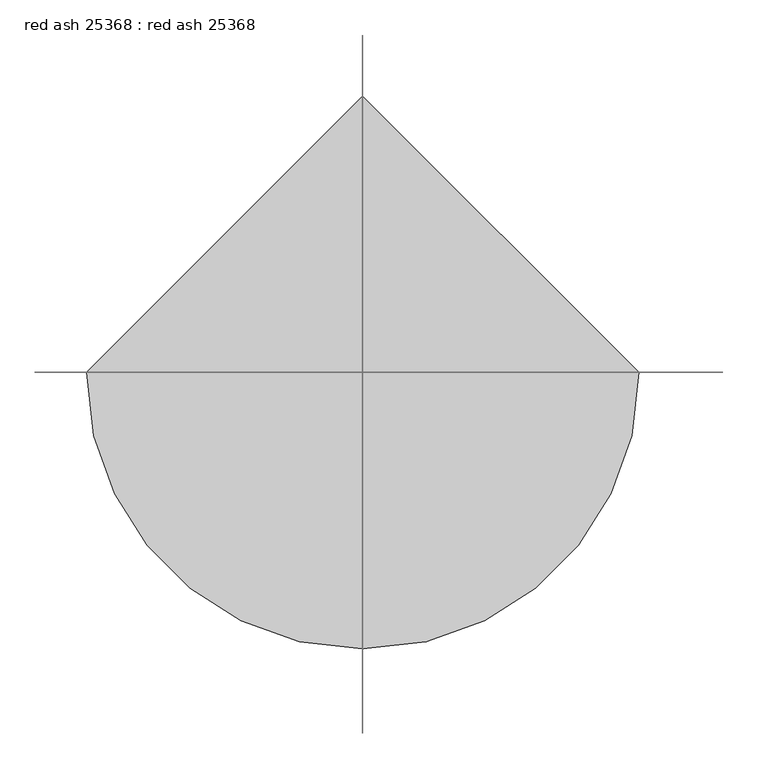
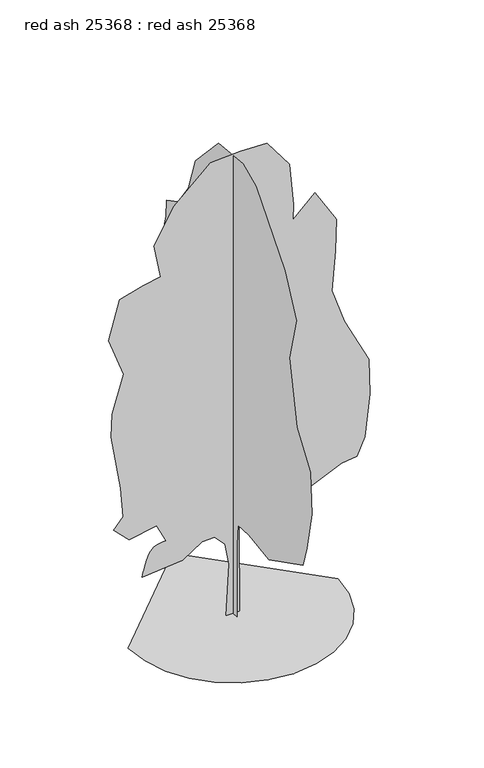
"""IFC4 building model written with IfcOpenShell, lengths in millimetres: proxy geometry, red ash 25368 : red ash 25368."""

import ifcopenshell
import ifcopenshell.guid

model = None  # the IFC model being written
_history = None  # IfcOwnerHistory: only IFC2X3 demands one
_inside = {}  # id of a spatial element -> (the spatial element, [elements in it])
_under = {}  # id of a project, library or spatial element -> (it, [spatial elements below it])
_declared = {}  # id of a project -> (the project, [libraries it declares])
_typed = {}  # id of a type object -> (the type object, [elements of that type])
_made_of = {}  # id of a material, layer set ... -> (it, [elements and type objects made of it])


def new_model(schema):
    """Start an empty IFC model of exactly this schema.

    Asked for "IFC4X3", IfcOpenShell would pick the latest addendum, in which some entities
    have other attributes; the version numbers below select the first issue.
    IFC2X3 requires an IfcOwnerHistory on every rooted entity: one is made here for all.
    """
    global model, _history
    if schema == "IFC4X3":
        model = ifcopenshell.file(schema_version=(4, 3, 0, 0))
    else:
        model = ifcopenshell.file(schema=schema)
    _inside.clear()
    _under.clear()
    _declared.clear()
    _typed.clear()
    _made_of.clear()
    _history = None
    if model.schema == "IFC2X3":
        org = make("IfcOrganization", Name="unknown")
        user = make(
            "IfcPersonAndOrganization",
            ThePerson=make("IfcPerson", FamilyName="unknown"),
            TheOrganization=org,
        )
        app = make(
            "IfcApplication",
            ApplicationDeveloper=org,
            Version="unknown",
            ApplicationFullName="unknown",
            ApplicationIdentifier="unknown",
        )
        _history = make(
            "IfcOwnerHistory",
            OwningUser=user,
            OwningApplication=app,
            ChangeAction="ADDED",
            CreationDate=0,
        )
    return model


def make(cls, **values):
    """One entity of the class cls with the attributes given. An attribute that is None is left unset."""
    return model.create_entity(
        cls, **{name: value for name, value in values.items() if value is not None}
    )


def rooted(cls, **values):
    """An entity with a GlobalId (a new one), such as an element, a storey or a relation."""
    return make(cls, GlobalId=ifcopenshell.guid.new(), OwnerHistory=_history, **values)


def si_unit(unit_type, name, prefix=None):
    """IfcSIUnit, for example si_unit("LENGTHUNIT", "METRE", prefix="MILLI")."""
    return make("IfcSIUnit", UnitType=unit_type, Prefix=prefix, Name=name)


def assignment(units):
    """IfcUnitAssignment: the units of a project."""
    return None if units is None else make("IfcUnitAssignment", Units=units)


def point(xyz):
    """IfcCartesianPoint."""
    return None if xyz is None else make("IfcCartesianPoint", Coordinates=xyz)


def direction(xyz):
    """IfcDirection."""
    return None if xyz is None else make("IfcDirection", DirectionRatios=xyz)


def frame(location, z_axis=None, x_axis=None):
    """IfcAxis2Placement3D, a coordinate frame: its origin and axes. An axis left out is left unset."""
    return make(
        "IfcAxis2Placement3D",
        Location=point(location),
        Axis=direction(z_axis),
        RefDirection=direction(x_axis),
    )


def origin():
    """The frame at (0, 0, 0) with its axes left unset."""
    return frame((0.0, 0.0, 0.0))


def place(relative_to, where):
    """IfcLocalPlacement: puts the frame where relative to a parent placement (None: the world)."""
    return make(
        "IfcLocalPlacement", PlacementRelTo=relative_to, RelativePlacement=where
    )


def context(
    kind, dimensions, precision=None, world=None, true_north=None, identifier=None
):
    """IfcGeometricRepresentationContext, for example the 3D "Model" context."""
    return make(
        "IfcGeometricRepresentationContext",
        ContextIdentifier=identifier,
        ContextType=kind,
        CoordinateSpaceDimension=dimensions,
        Precision=precision,
        WorldCoordinateSystem=world,
        TrueNorth=true_north,
    )


def project(units=None, contexts=None):
    """IfcProject with its units and contexts."""
    return rooted(
        "IfcProject",
        Name="project",
        RepresentationContexts=contexts,
        UnitsInContext=assignment(units),
    )


def spatial(cls, under=None, at=None, **own):
    """A site, building, storey or space (cls), placed at a placement, below another one or the project."""
    s = rooted(cls, ObjectPlacement=at, **own)
    if under is not None:
        _under.setdefault(under.id(), (under, []))[1].append(s)
    return s


def point_list(points):
    """IfcCartesianPointList2D or 3D."""
    cls = (
        "IfcCartesianPointList2D" if len(points[0]) == 2 else "IfcCartesianPointList3D"
    )
    return make(cls, CoordList=points)


def triangles(points, corners, closed=None, point_numbers=None):
    """IfcTriangulatedFaceSet: each triangle names its three corners, points numbered from 1."""
    return make(
        "IfcTriangulatedFaceSet",
        Coordinates=point_list(points),
        Closed=closed,
        CoordIndex=corners,
        PnIndex=point_numbers,
    )


def shape(context_of_items, identifier, shape_type, items):
    """IfcShapeRepresentation: the items that make up one representation, for example the "Body"."""
    return make(
        "IfcShapeRepresentation",
        ContextOfItems=context_of_items,
        RepresentationIdentifier=identifier,
        RepresentationType=shape_type,
        Items=items,
    )


def source(mapping_origin, context_of_items, identifier, shape_type, items):
    """IfcRepresentationMap: a shape defined once, which mapped items show again and again."""
    return make(
        "IfcRepresentationMap",
        MappingOrigin=mapping_origin,
        MappedRepresentation=shape(context_of_items, identifier, shape_type, items),
    )


def transform(
    local_origin,
    x_axis=None,
    y_axis=None,
    z_axis=None,
    scale=None,
    scale2=None,
    scale3=None,
    uniform=True,
):
    """IfcCartesianTransformationOperator3D, or its non-uniform kind. x_axis, y_axis, z_axis: its Axis1, 2, 3."""
    if uniform:
        return make(
            "IfcCartesianTransformationOperator3D",
            Axis1=direction(x_axis),
            Axis2=direction(y_axis),
            LocalOrigin=point(local_origin),
            Scale=scale,
            Axis3=direction(z_axis),
        )
    return make(
        "IfcCartesianTransformationOperator3DnonUniform",
        Axis1=direction(x_axis),
        Axis2=direction(y_axis),
        LocalOrigin=point(local_origin),
        Scale=scale,
        Axis3=direction(z_axis),
        Scale2=scale2,
        Scale3=scale3,
    )


def mapped(mapping_source, mapping_target):
    """IfcMappedItem: shows the shape of a source again, moved by a transform."""
    return make(
        "IfcMappedItem", MappingSource=mapping_source, MappingTarget=mapping_target
    )


def made_of(thing, what):
    """Note that an element or type object is made of a material, layer set ...; save() writes the relation."""
    if what is not None:
        _made_of.setdefault(what.id(), (what, []))[1].append(thing)
    return thing


def element(
    cls,
    number,
    at=None,
    inside=None,
    cuts=None,
    type_object=None,
    material=None,
    context=None,
    identifier="Body",
    shape_type=None,
    held_by="IfcProductDefinitionShape",
    body=None,
    shapes=None,
    **own,
):
    """One element of the class cls, such as IfcWall. Its Tag is "e" and its number.

    at: its placement. inside: the storey or other place that contains it. cuts: it is an
    opening in that element (IfcRelVoidsElement). A single representation is given by context,
    identifier, shape_type and body (its items); several are given by shapes. held_by: the class
    of the entity that holds the representations. save() writes the other relations.
    """
    e = rooted(cls, Tag="e%d" % number, ObjectPlacement=at, **own)
    if body is not None:
        shapes = [shape(context, identifier, shape_type, body)]
    if shapes is not None:
        e.Representation = make(held_by, Representations=shapes)
    if inside is not None:
        _inside.setdefault(inside.id(), (inside, []))[1].append(e)
    if cuts is not None:
        rooted(
            "IfcRelVoidsElement", RelatingBuildingElement=cuts, RelatedOpeningElement=e
        )
    if type_object is not None:
        _typed.setdefault(type_object.id(), (type_object, []))[1].append(e)
    return made_of(e, material)


def aggregate(whole, parts):
    """IfcRelAggregates: a whole, such as a stair, and the parts it consists of."""
    return rooted("IfcRelAggregates", RelatingObject=whole, RelatedObjects=parts)


def save(model, path):
    """Write the relations noted so far, then the file.

    IfcRelAggregates (storeys below a building ...), IfcRelContainedInSpatialStructure (elements
    in a storey), IfcRelDefinesByType, IfcRelAssociatesMaterial and IfcRelDeclares: one each for
    every whole, place, type object, material and project.
    """
    for whole, parts in _under.values():
        aggregate(whole, parts)
    for where, things in _inside.values():
        rooted(
            "IfcRelContainedInSpatialStructure",
            RelatedElements=things,
            RelatingStructure=where,
        )
    for kind, things in _typed.values():
        rooted("IfcRelDefinesByType", RelatedObjects=things, RelatingType=kind)
    for what, things in _made_of.values():
        rooted("IfcRelAssociatesMaterial", RelatedObjects=things, RelatingMaterial=what)
    for by, libraries in _declared.values():
        rooted("IfcRelDeclares", RelatingContext=by, RelatedDefinitions=libraries)
    model.write(path)


def red_ash_25368_red_ash_25368_14781bec(model_context):
    return source(origin(), model_context, "Body", "Tessellation", [
        triangles([(-1644.9525009, 0.0, 6.19e-05), (-1601.4651844, -376.9143482, 6.19e-05), (-1477.6144592, -723.0498339, 6.19e-05), (-1283.3164352, -1028.4894024, 6.19e-05), (-1028.4894751, -1283.3165806, 6.19e-05), (-723.0496885, -1477.6140232, 6.19e-05), (-376.9141665, -1601.4651844, 6.19e-05), (7.19e-05, -1644.9525009, 6.19e-05), (376.9143846, -1601.4651844, 6.19e-05), (723.0499065, -1477.6143139, 6.19e-05), (1028.4894751, -1283.3164352, 6.19e-05), (1283.3168713, -1028.4894751, 6.19e-05), (1477.6141685, -723.0496159, 6.19e-05), (1601.4651844, -376.9140939, 6.19e-05), (1644.9525009, 0.0001438, 6.19e-05), (-0.0002157, 1644.9525009, 6.19e-05), (-1.07e-05, -102.8462569, 0.0), (2.5e-05, -101.2467179, 1194.554048), (3.23e-05, -129.8819613, 1537.8029366), (7e-07, -438.8253948, 1558.1655018), (-5.78e-05, -976.3912743, 1478.3068588), (-0.0001405, -1903.692667, 1948.6771305), (-0.0001413, -2011.2060173, 2298.095192), (-0.0001361, -2145.5975235, 2943.1744217), (-0.0001119, -2105.2803623, 3615.1319527), (-5.81e-05, -1740.3819958, 4141.0172951), (-5.5e-06, -1527.3986298, 5160.6350006), (-3.5e-06, -1715.5451397, 5886.3488434), (4.79e-05, -1406.4449661, 6531.4286545), (0.0001569, -626.9743755, 7458.7301926), (0.0001985, -273.2007115, 7618.1942963), (0.0002662, 394.4016166, 7552.8046829), (0.0003121, 1026.0418774, 6880.8468613), (0.0003149, 1214.190204, 6316.4022446), (0.0003323, 1496.411277, 5913.2274353), (0.0003598, 1805.5131947, 5751.9582092), (0.0003531, 1818.9521999, 5483.1746155), (0.0003523, 1899.587249, 5174.0742966), (0.0003275, 1765.1957428, 4811.2170845), (0.0003297, 1886.1480984, 4461.7991684), (0.0003279, 2007.1004539, 3977.9897461), (0.0003211, 1980.222298, 3843.5979492), (0.0002877, 1751.7567375, 3521.0580437), (0.0002729, 1737.3115437, 3077.5662186), (0.0002632, 1724.8782909, 2795.3439102), (0.0002542, 1738.3174416, 2445.9262848), (0.0002412, 1751.7568829, 1962.1167171), (0.0002172, 1563.6084835, 1814.2857697), (0.0001807, 1214.1907127, 1814.2857697), (0.0001827, 1375.4605202, 1317.0371967), (0.0001715, 1348.4951603, 1034.8845062), (0.0001516, 1103.0310734, 1227.8363914), (9.86e-05, 629.4626684, 1106.7075932), (9.8e-05, 551.7118183, 1357.0609165), (6.29e-05, 215.9127657, 1354.0025276), (5.03e-05, 130.8012366, 1228.3346169), (3.27e-05, 79.5493323, 818.2831198), (1.17e-05, 112.1660096, 1.28e-05), (-110.870867, 4.8e-06, 4.46e-05), (-66.7114758, -9.64e-05, 833.5016676), (-129.3072962, -0.000136, 1187.9435503), (-290.7878647, -0.00015, 1365.31768), (-483.6364677, -0.0001408, 1358.6964272), (-796.2678211, -0.000103, 1155.7673166), (-1427.9080456, -6.9e-05, 1102.0108595), (-1419.1706429, -7.35e-05, 1136.7646975), (-1409.8454853, -7.82e-05, 1172.6938271), (-1399.3449635, -8.32e-05, 1210.9736853), (-1387.0813225, -8.87e-05, 1252.7803631), (-1372.4668076, -9.49e-05, 1299.2876987), (-1354.9136639, -0.0001019, 1351.6733093), (-1333.8341366, -0.0001099, 1411.1111057), (-1307.2693336, -0.0001176, 1466.2392815), (-1274.3570984, -0.0001239, 1506.556588), (-1236.1555058, -0.0001289, 1534.5316246), (-1193.7220493, -0.0001329, 1552.6338627), (-1148.1152401, -0.0001362, 1563.3300121), (-1100.3923536, -0.000139, 1569.0895443), (-1051.6116829, -0.0001415, 1572.3809132), (-1199.4421944, -0.0001703, 1868.0423721), (-1629.4953049, -0.0001418, 1787.4073231), (-1871.3997253, -0.0001601, 2029.3124702), (-1723.5690685, -0.0001874, 2204.0214283), (-1763.886375, -0.0002433, 2687.8309959), (-1911.7170319, -0.0003442, 3588.2539421), (-1898.4807758, -0.0003892, 3961.1654823), (-1719.9175472, -0.0004688, 4563.3255295), (-1952.0346291, -0.0005347, 5200.9523071), (-1777.3253803, -0.000616, 5819.1535263), (-1414.4687496, -0.0006447, 5926.6667313), (-1138.413216, -0.0006626, 5975.3625961), (-1239.7599369, -0.0007228, 6517.9893585), (-930.6591093, -0.000802, 7068.9952606), (-352.7753057, -0.0008898, 7593.1219894), (117.5946844, -0.0009135, 7620.0), (534.2087442, -0.0009301, 7606.5601227), (883.626733, -0.0008893, 7136.1905777), (947.8720848, -0.00081, 6447.5180786), (938.6469212, -0.0007795, 6194.9695404), (1286.8011063, -0.0008333, 6517.9893585), (1622.7800171, -0.0007823, 5966.9840378), (1609.3410118, -0.0007196, 5446.5094116), (1549.4574577, -0.00064, 4800.6520317), (1743.7323727, -0.0005809, 4233.3331718), (2131.7640656, -0.0005067, 3469.1978371), (2144.1354034, -0.0004386, 2892.8094727), (2066.2719875, -0.0003531, 2204.021283), (1945.319632, -0.0003141, 1921.7989746), (1703.4147755, -0.0003004, 1894.9206734), (1233.0446491, -0.0002542, 1679.8941181), (816.4305439, -0.0002007, 1384.2328045), (257.4765441, -0.0002049, 1624.5688614), (93.0508701, -0.0001766, 1447.6347485), (104.1552431, -4.6e-06, 3.52e-05)], [[15, 16, 1], [14, 15, 1], [14, 1, 2], [13, 14, 2], [13, 2, 3], [13, 3, 4], [12, 13, 4], [11, 12, 4], [11, 4, 5], [11, 5, 6], [11, 6, 7], [11, 7, 8], [11, 8, 9], [11, 9, 10], [50, 51, 52], [57, 58, 17], [57, 17, 18], [56, 57, 18], [56, 18, 19], [55, 56, 19], [49, 50, 52], [52, 53, 54], [49, 52, 54], [35, 36, 37], [46, 47, 48], [46, 48, 49], [21, 22, 23], [20, 21, 23], [20, 23, 24], [20, 24, 25], [20, 25, 26], [19, 20, 26], [19, 26, 27], [45, 46, 49], [31, 32, 33], [30, 31, 33], [29, 30, 33], [29, 33, 34], [28, 29, 34], [27, 28, 34], [19, 27, 34], [19, 34, 35], [19, 35, 37], [19, 37, 38], [19, 38, 39], [19, 39, 40], [19, 40, 41], [19, 41, 42], [19, 42, 43], [19, 43, 44], [19, 44, 45], [19, 45, 49], [19, 49, 54], [55, 19, 54], [64, 65, 66], [64, 66, 67], [64, 67, 68], [99, 100, 101], [64, 68, 69], [64, 69, 70], [64, 70, 71], [114, 59, 60], [113, 114, 60], [113, 60, 61], [113, 61, 62], [64, 71, 72], [64, 72, 73], [64, 73, 74], [64, 74, 75], [64, 75, 76], [64, 76, 77], [64, 77, 78], [64, 78, 79], [63, 64, 79], [81, 82, 83], [80, 81, 83], [99, 101, 102], [107, 108, 109], [110, 111, 112], [88, 89, 90], [87, 88, 90], [87, 90, 91], [80, 83, 84], [95, 96, 97], [95, 97, 98], [94, 95, 98], [93, 94, 98], [92, 93, 98], [91, 92, 98], [91, 98, 99], [87, 91, 99], [87, 99, 102], [87, 102, 103], [87, 103, 104], [86, 87, 104], [85, 86, 104], [84, 85, 104], [80, 84, 104], [80, 104, 105], [80, 105, 106], [80, 106, 107], [80, 107, 109], [80, 109, 110], [80, 110, 112], [79, 80, 112], [63, 79, 112], [62, 63, 112], [113, 62, 112]], closed=False),
    ])


if __name__ == "__main__":
    model = new_model("IFC4")
    model_context = context("Model", 3, world=origin())
    ifc_project = project(units=[si_unit("LENGTHUNIT", "METRE", prefix="MILLI")], contexts=[model_context])
    site = spatial("IfcSite", under=ifc_project)
    building = spatial("IfcBuilding", under=site)
    placement = place(None, origin())
    red_ash_25368_red_ash_25368_shape = red_ash_25368_red_ash_25368_14781bec(model_context)
    element("IfcBuildingElementProxy", 1, Name="red ash 25368 : red ash 25368", ObjectType="red ash 25368 : red ash 25368", at=placement, inside=building, context=model_context, shape_type="MappedRepresentation", body=[
        mapped(red_ash_25368_red_ash_25368_shape, transform((0.0, 0.0, 0.0), x_axis=(1.0, 0.0, 0.0), y_axis=(0.0, 1.0, 0.0), z_axis=(0.0, 0.0, 1.0))),
    ])
    save(model, "model.ifc")

# Revit data of these elements
# Type "red ash 25368 : red ash 25368"
#   built-in parameter 1005195 = "RPC-8-G3GR-497X-PHW5-6"
#   Height = 0
